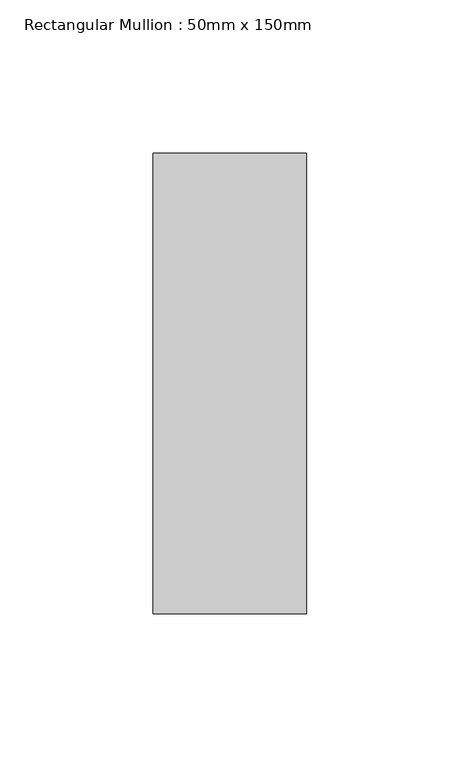
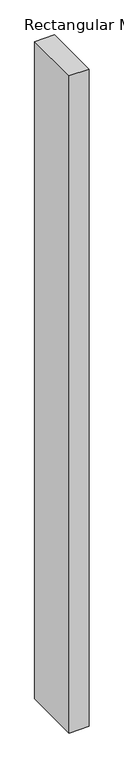
"""IFC4 building model written with IfcOpenShell, lengths in millimetres: member geometry, Rectangular Mullion : 50mm x 150mm."""

from ifc_helpers import new_model, si_unit, frame, origin, place, context, project, spatial, polyline, outline, extrude, source, transform, mapped, element, save


def rectangular_mullion_50mm_x_150mm_c21f2d45(model_context):
    return source(origin(), model_context, "Body", "SweptSolid", [
        extrude(outline(polyline([(0.0, 75.0), (0.0, -75.0), (-50.0, -75.0), (-50.0, 75.0), (0.0, 75.0)])), frame((0.0, 0.0, -1740.2939092), z_axis=(0.0, 0.0, 1.0), x_axis=(1.0, 0.0, 0.0)), (0.0, 0.0, 1.0), 1740.2939092),
    ])


if __name__ == "__main__":
    model = new_model("IFC4")
    model_context = context("Model", 3, world=origin())
    ifc_project = project(units=[si_unit("LENGTHUNIT", "METRE", prefix="MILLI")], contexts=[model_context])
    site = spatial("IfcSite", under=ifc_project)
    building = spatial("IfcBuilding", under=site)
    placement = place(None, origin())
    rectangular_mullion_50mm_x_150mm_shape = rectangular_mullion_50mm_x_150mm_c21f2d45(model_context)
    element("IfcMember", 1, ObjectType="Rectangular Mullion : 50mm x 150mm", at=placement, inside=building, context=model_context, shape_type="MappedRepresentation", body=[
        mapped(rectangular_mullion_50mm_x_150mm_shape, transform((0.0, 0.0, 0.0), x_axis=(1.0, 0.0, 0.0), y_axis=(0.0, 1.0, 0.0), z_axis=(0.0, 0.0, 1.0))),
    ])
    save(model, "model.ifc")

# Revit data of these elements
# Type "Rectangular Mullion : 50mm x 150mm"
#   built-in parameter 1007304 = 0.492126 (stored number, unit not read)
#   built-in parameter 1007301 = 0.082021 (stored number, unit not read)
#   built-in parameter 1007300 = 0.082021 (stored number, unit not read)
# Element 1 (IfcMember, "Rectangular Mullion : 50mm x 150mm")
#   Materials on its faces: "Aluminum"
# Materials
#   "Aluminum": class "Metal", colour RGB 244 244 244, transparency 0, Description = "Aluminum 6061", Cost = 0
